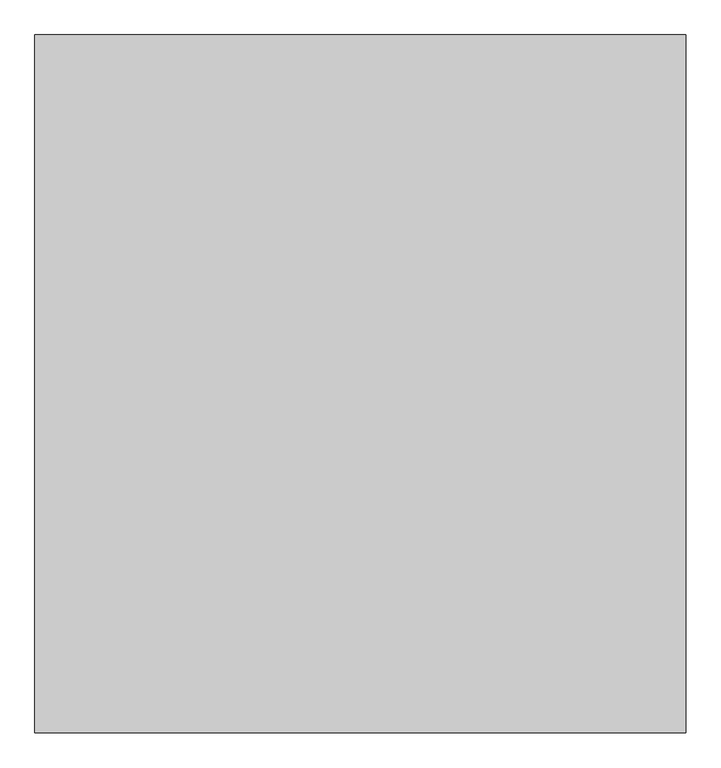
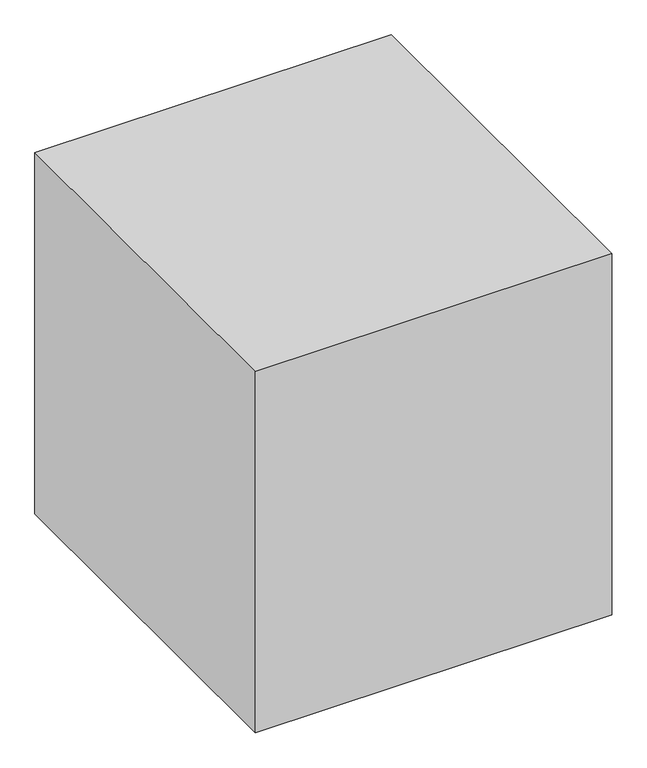
"""IFC4 building model written with IfcOpenShell, lengths in millimetres: proxy geometry, Space Planning Box_hec : Space Planning Box_hec."""

import ifcopenshell
import ifcopenshell.guid

model = None  # the IFC model being written
_history = None  # IfcOwnerHistory: only IFC2X3 demands one
_inside = {}  # id of a spatial element -> (the spatial element, [elements in it])
_under = {}  # id of a project, library or spatial element -> (it, [spatial elements below it])
_declared = {}  # id of a project -> (the project, [libraries it declares])
_typed = {}  # id of a type object -> (the type object, [elements of that type])
_made_of = {}  # id of a material, layer set ... -> (it, [elements and type objects made of it])


def new_model(schema):
    """Start an empty IFC model of exactly this schema.

    Asked for "IFC4X3", IfcOpenShell would pick the latest addendum, in which some entities
    have other attributes; the version numbers below select the first issue.
    IFC2X3 requires an IfcOwnerHistory on every rooted entity: one is made here for all.
    """
    global model, _history
    if schema == "IFC4X3":
        model = ifcopenshell.file(schema_version=(4, 3, 0, 0))
    else:
        model = ifcopenshell.file(schema=schema)
    _inside.clear()
    _under.clear()
    _declared.clear()
    _typed.clear()
    _made_of.clear()
    _history = None
    if model.schema == "IFC2X3":
        org = make("IfcOrganization", Name="unknown")
        user = make(
            "IfcPersonAndOrganization",
            ThePerson=make("IfcPerson", FamilyName="unknown"),
            TheOrganization=org,
        )
        app = make(
            "IfcApplication",
            ApplicationDeveloper=org,
            Version="unknown",
            ApplicationFullName="unknown",
            ApplicationIdentifier="unknown",
        )
        _history = make(
            "IfcOwnerHistory",
            OwningUser=user,
            OwningApplication=app,
            ChangeAction="ADDED",
            CreationDate=0,
        )
    return model


def make(cls, **values):
    """One entity of the class cls with the attributes given. An attribute that is None is left unset."""
    return model.create_entity(
        cls, **{name: value for name, value in values.items() if value is not None}
    )


def rooted(cls, **values):
    """An entity with a GlobalId (a new one), such as an element, a storey or a relation."""
    return make(cls, GlobalId=ifcopenshell.guid.new(), OwnerHistory=_history, **values)


def si_unit(unit_type, name, prefix=None):
    """IfcSIUnit, for example si_unit("LENGTHUNIT", "METRE", prefix="MILLI")."""
    return make("IfcSIUnit", UnitType=unit_type, Prefix=prefix, Name=name)


def assignment(units):
    """IfcUnitAssignment: the units of a project."""
    return None if units is None else make("IfcUnitAssignment", Units=units)


def point(xyz):
    """IfcCartesianPoint."""
    return None if xyz is None else make("IfcCartesianPoint", Coordinates=xyz)


def direction(xyz):
    """IfcDirection."""
    return None if xyz is None else make("IfcDirection", DirectionRatios=xyz)


def frame(location, z_axis=None, x_axis=None):
    """IfcAxis2Placement3D, a coordinate frame: its origin and axes. An axis left out is left unset."""
    return make(
        "IfcAxis2Placement3D",
        Location=point(location),
        Axis=direction(z_axis),
        RefDirection=direction(x_axis),
    )


def origin():
    """The frame at (0, 0, 0) with its axes left unset."""
    return frame((0.0, 0.0, 0.0))


def origin_with_axes():
    """The frame at (0, 0, 0) with the z axis (0, 0, 1) and the x axis (1, 0, 0) written out."""
    return frame((0.0, 0.0, 0.0), z_axis=(0.0, 0.0, 1.0), x_axis=(1.0, 0.0, 0.0))


def place(relative_to, where):
    """IfcLocalPlacement: puts the frame where relative to a parent placement (None: the world)."""
    return make(
        "IfcLocalPlacement", PlacementRelTo=relative_to, RelativePlacement=where
    )


def context(
    kind, dimensions, precision=None, world=None, true_north=None, identifier=None
):
    """IfcGeometricRepresentationContext, for example the 3D "Model" context."""
    return make(
        "IfcGeometricRepresentationContext",
        ContextIdentifier=identifier,
        ContextType=kind,
        CoordinateSpaceDimension=dimensions,
        Precision=precision,
        WorldCoordinateSystem=world,
        TrueNorth=true_north,
    )


def project(units=None, contexts=None):
    """IfcProject with its units and contexts."""
    return rooted(
        "IfcProject",
        Name="project",
        RepresentationContexts=contexts,
        UnitsInContext=assignment(units),
    )


def spatial(cls, under=None, at=None, **own):
    """A site, building, storey or space (cls), placed at a placement, below another one or the project."""
    s = rooted(cls, ObjectPlacement=at, **own)
    if under is not None:
        _under.setdefault(under.id(), (under, []))[1].append(s)
    return s


def polyline(points):
    """IfcPolyline through the points."""
    return make("IfcPolyline", Points=[point(p) for p in points])


def outline(outer, holes=None, kind="AREA"):
    """IfcArbitraryClosedProfileDef: a profile drawn as a closed curve; with holes, ...WithVoids."""
    if holes is None:
        return make("IfcArbitraryClosedProfileDef", ProfileType=kind, OuterCurve=outer)
    return make(
        "IfcArbitraryProfileDefWithVoids",
        ProfileType=kind,
        OuterCurve=outer,
        InnerCurves=holes,
    )


def extrude(swept, where, along, depth):
    """IfcExtrudedAreaSolid: the profile swept, set in the frame where, extruded along a direction by depth."""
    return make(
        "IfcExtrudedAreaSolid",
        SweptArea=swept,
        Position=where,
        ExtrudedDirection=direction(along),
        Depth=depth,
    )


def shape(context_of_items, identifier, shape_type, items):
    """IfcShapeRepresentation: the items that make up one representation, for example the "Body"."""
    return make(
        "IfcShapeRepresentation",
        ContextOfItems=context_of_items,
        RepresentationIdentifier=identifier,
        RepresentationType=shape_type,
        Items=items,
    )


def source(mapping_origin, context_of_items, identifier, shape_type, items):
    """IfcRepresentationMap: a shape defined once, which mapped items show again and again."""
    return make(
        "IfcRepresentationMap",
        MappingOrigin=mapping_origin,
        MappedRepresentation=shape(context_of_items, identifier, shape_type, items),
    )


def transform(
    local_origin,
    x_axis=None,
    y_axis=None,
    z_axis=None,
    scale=None,
    scale2=None,
    scale3=None,
    uniform=True,
):
    """IfcCartesianTransformationOperator3D, or its non-uniform kind. x_axis, y_axis, z_axis: its Axis1, 2, 3."""
    if uniform:
        return make(
            "IfcCartesianTransformationOperator3D",
            Axis1=direction(x_axis),
            Axis2=direction(y_axis),
            LocalOrigin=point(local_origin),
            Scale=scale,
            Axis3=direction(z_axis),
        )
    return make(
        "IfcCartesianTransformationOperator3DnonUniform",
        Axis1=direction(x_axis),
        Axis2=direction(y_axis),
        LocalOrigin=point(local_origin),
        Scale=scale,
        Axis3=direction(z_axis),
        Scale2=scale2,
        Scale3=scale3,
    )


def mapped(mapping_source, mapping_target):
    """IfcMappedItem: shows the shape of a source again, moved by a transform."""
    return make(
        "IfcMappedItem", MappingSource=mapping_source, MappingTarget=mapping_target
    )


def made_of(thing, what):
    """Note that an element or type object is made of a material, layer set ...; save() writes the relation."""
    if what is not None:
        _made_of.setdefault(what.id(), (what, []))[1].append(thing)
    return thing


def element(
    cls,
    number,
    at=None,
    inside=None,
    cuts=None,
    type_object=None,
    material=None,
    context=None,
    identifier="Body",
    shape_type=None,
    held_by="IfcProductDefinitionShape",
    body=None,
    shapes=None,
    **own,
):
    """One element of the class cls, such as IfcWall. Its Tag is "e" and its number.

    at: its placement. inside: the storey or other place that contains it. cuts: it is an
    opening in that element (IfcRelVoidsElement). A single representation is given by context,
    identifier, shape_type and body (its items); several are given by shapes. held_by: the class
    of the entity that holds the representations. save() writes the other relations.
    """
    e = rooted(cls, Tag="e%d" % number, ObjectPlacement=at, **own)
    if body is not None:
        shapes = [shape(context, identifier, shape_type, body)]
    if shapes is not None:
        e.Representation = make(held_by, Representations=shapes)
    if inside is not None:
        _inside.setdefault(inside.id(), (inside, []))[1].append(e)
    if cuts is not None:
        rooted(
            "IfcRelVoidsElement", RelatingBuildingElement=cuts, RelatedOpeningElement=e
        )
    if type_object is not None:
        _typed.setdefault(type_object.id(), (type_object, []))[1].append(e)
    return made_of(e, material)


def aggregate(whole, parts):
    """IfcRelAggregates: a whole, such as a stair, and the parts it consists of."""
    return rooted("IfcRelAggregates", RelatingObject=whole, RelatedObjects=parts)


def save(model, path):
    """Write the relations noted so far, then the file.

    IfcRelAggregates (storeys below a building ...), IfcRelContainedInSpatialStructure (elements
    in a storey), IfcRelDefinesByType, IfcRelAssociatesMaterial and IfcRelDeclares: one each for
    every whole, place, type object, material and project.
    """
    for whole, parts in _under.values():
        aggregate(whole, parts)
    for where, things in _inside.values():
        rooted(
            "IfcRelContainedInSpatialStructure",
            RelatedElements=things,
            RelatingStructure=where,
        )
    for kind, things in _typed.values():
        rooted("IfcRelDefinesByType", RelatedObjects=things, RelatingType=kind)
    for what, things in _made_of.values():
        rooted("IfcRelAssociatesMaterial", RelatedObjects=things, RelatingMaterial=what)
    for by, libraries in _declared.values():
        rooted("IfcRelDeclares", RelatingContext=by, RelatedDefinitions=libraries)
    model.write(path)


def generic_models_ec17d728(model_context):
    return source(origin(), model_context, "Body", "SweptSolid", [
        extrude(outline(polyline([(2800.0, 3000.0), (2800.0, -3000.0), (-2800.0, -3000.0), (-2800.0, 3000.0), (2800.0, 3000.0)])), origin_with_axes(), (0.0, 0.0, 1.0), 6000.0),
    ])


if __name__ == "__main__":
    model = new_model("IFC4")
    model_context = context("Model", 3, world=origin())
    ifc_project = project(units=[si_unit("LENGTHUNIT", "METRE", prefix="MILLI")], contexts=[model_context])
    site = spatial("IfcSite", under=ifc_project)
    building = spatial("IfcBuilding", under=site)
    placement = place(None, origin())
    generic_models_shape = generic_models_ec17d728(model_context)
    element("IfcBuildingElementProxy", 1, Name="Space Planning Box_hec : Space Planning Box_hec", ObjectType="Space Planning Box_hec : Space Planning Box_hec", at=placement, inside=building, context=model_context, shape_type="MappedRepresentation", body=[
        mapped(generic_models_shape, transform((0.0, 0.0, 0.0), x_axis=(1.0, 0.0, 0.0), y_axis=(0.0, 1.0, 0.0), z_axis=(0.0, 0.0, 1.0))),
    ])
    save(model, "model.ifc")

# Revit data of these elements
# Type "Space Planning Box_hec : Space Planning Box_hec"
#   Type Comments = "..."
#   Room Name [instance default] = "?"
#   Interior Finish [instance default] = ""
#   Exterior Finish [instance default] = ""
#   Department [instance default] = ""
#   Assembly Code = "..."
#   Width [instance default] = 1524 mm
#   Program Area [instance default] = 0.00 m²
#   Length [instance default] = 1524 mm
#   Height [instance default] = 1524 mm
#   Area [instance default] = 2.32258 m²
#   Fill Color [instance default] = Cyan
#   Default Elevation = 0
# Element 1 (IfcBuildingElementProxy, "Space Planning Box_hec : Space Planning Box_hec")
#   Room Name = "Locker Room (M)"
#   Interior Finish = "IF2-1"
#   Exterior Finish = "EF1"
#   Department = "AR"
#   Width = 5600 mm
#   Program Area = 31.50 m²
#   Length = 6000 mm
#   Height = 6000 mm
#   Area = 33.60 m²
#   Fill Color = Lavender
#   Materials on its faces: "Lavender"
# Materials
#   "Cyan": class "Generic", colour RGB 0 255 255, transparency 0.2, Cost = 0
#   "Lavender": class "Generic", colour RGB 186 85 211, transparency 0.2, Cost = 0
